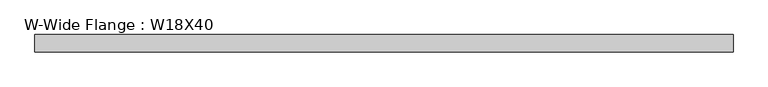
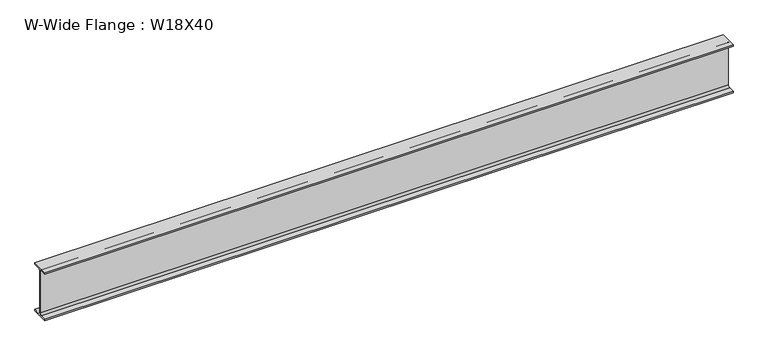
"""IFC4 building model written with IfcOpenShell, lengths in millimetres: beam geometry, W-Wide Flange : W18X40."""

import ifcopenshell
import ifcopenshell.guid

model = None  # the IFC model being written
_history = None  # IfcOwnerHistory: only IFC2X3 demands one
_inside = {}  # id of a spatial element -> (the spatial element, [elements in it])
_under = {}  # id of a project, library or spatial element -> (it, [spatial elements below it])
_declared = {}  # id of a project -> (the project, [libraries it declares])
_typed = {}  # id of a type object -> (the type object, [elements of that type])
_made_of = {}  # id of a material, layer set ... -> (it, [elements and type objects made of it])


def new_model(schema):
    """Start an empty IFC model of exactly this schema.

    Asked for "IFC4X3", IfcOpenShell would pick the latest addendum, in which some entities
    have other attributes; the version numbers below select the first issue.
    IFC2X3 requires an IfcOwnerHistory on every rooted entity: one is made here for all.
    """
    global model, _history
    if schema == "IFC4X3":
        model = ifcopenshell.file(schema_version=(4, 3, 0, 0))
    else:
        model = ifcopenshell.file(schema=schema)
    _inside.clear()
    _under.clear()
    _declared.clear()
    _typed.clear()
    _made_of.clear()
    _history = None
    if model.schema == "IFC2X3":
        org = make("IfcOrganization", Name="unknown")
        user = make(
            "IfcPersonAndOrganization",
            ThePerson=make("IfcPerson", FamilyName="unknown"),
            TheOrganization=org,
        )
        app = make(
            "IfcApplication",
            ApplicationDeveloper=org,
            Version="unknown",
            ApplicationFullName="unknown",
            ApplicationIdentifier="unknown",
        )
        _history = make(
            "IfcOwnerHistory",
            OwningUser=user,
            OwningApplication=app,
            ChangeAction="ADDED",
            CreationDate=0,
        )
    return model


def make(cls, **values):
    """One entity of the class cls with the attributes given. An attribute that is None is left unset."""
    return model.create_entity(
        cls, **{name: value for name, value in values.items() if value is not None}
    )


def rooted(cls, **values):
    """An entity with a GlobalId (a new one), such as an element, a storey or a relation."""
    return make(cls, GlobalId=ifcopenshell.guid.new(), OwnerHistory=_history, **values)


def si_unit(unit_type, name, prefix=None):
    """IfcSIUnit, for example si_unit("LENGTHUNIT", "METRE", prefix="MILLI")."""
    return make("IfcSIUnit", UnitType=unit_type, Prefix=prefix, Name=name)


def assignment(units):
    """IfcUnitAssignment: the units of a project."""
    return None if units is None else make("IfcUnitAssignment", Units=units)


def point(xyz):
    """IfcCartesianPoint."""
    return None if xyz is None else make("IfcCartesianPoint", Coordinates=xyz)


def direction(xyz):
    """IfcDirection."""
    return None if xyz is None else make("IfcDirection", DirectionRatios=xyz)


def frame(location, z_axis=None, x_axis=None):
    """IfcAxis2Placement3D, a coordinate frame: its origin and axes. An axis left out is left unset."""
    return make(
        "IfcAxis2Placement3D",
        Location=point(location),
        Axis=direction(z_axis),
        RefDirection=direction(x_axis),
    )


def frame_2d(location, x_axis=None):
    """IfcAxis2Placement2D, a coordinate frame in the plane: its origin and x axis."""
    return make(
        "IfcAxis2Placement2D", Location=point(location), RefDirection=direction(x_axis)
    )


def origin():
    """The frame at (0, 0, 0) with its axes left unset."""
    return frame((0.0, 0.0, 0.0))


def place(relative_to, where):
    """IfcLocalPlacement: puts the frame where relative to a parent placement (None: the world)."""
    return make(
        "IfcLocalPlacement", PlacementRelTo=relative_to, RelativePlacement=where
    )


def context(
    kind, dimensions, precision=None, world=None, true_north=None, identifier=None
):
    """IfcGeometricRepresentationContext, for example the 3D "Model" context."""
    return make(
        "IfcGeometricRepresentationContext",
        ContextIdentifier=identifier,
        ContextType=kind,
        CoordinateSpaceDimension=dimensions,
        Precision=precision,
        WorldCoordinateSystem=world,
        TrueNorth=true_north,
    )


def project(units=None, contexts=None):
    """IfcProject with its units and contexts."""
    return rooted(
        "IfcProject",
        Name="project",
        RepresentationContexts=contexts,
        UnitsInContext=assignment(units),
    )


def spatial(cls, under=None, at=None, **own):
    """A site, building, storey or space (cls), placed at a placement, below another one or the project."""
    s = rooted(cls, ObjectPlacement=at, **own)
    if under is not None:
        _under.setdefault(under.id(), (under, []))[1].append(s)
    return s


def polyline(points):
    """IfcPolyline through the points."""
    return make("IfcPolyline", Points=[point(p) for p in points])


def circle_curve(where, radius):
    """IfcCircle in the frame where."""
    return make("IfcCircle", Position=where, Radius=radius)


def trimmed(basis, trim1, trim2, sense, master):
    """IfcTrimmedCurve: the piece of a basis curve between two trims."""
    return make(
        "IfcTrimmedCurve",
        BasisCurve=basis,
        Trim1=trim1,
        Trim2=trim2,
        SenseAgreement=sense,
        MasterRepresentation=master,
    )


def segment(curve, same_sense, transition):
    """IfcCompositeCurveSegment."""
    return make(
        "IfcCompositeCurveSegment",
        Transition=transition,
        SameSense=same_sense,
        ParentCurve=curve,
    )


def composite_curve(segments, self_intersect=None):
    """IfcCompositeCurve: segments joined end to end."""
    return make("IfcCompositeCurve", Segments=segments, SelfIntersect=self_intersect)


def outline(outer, holes=None, kind="AREA"):
    """IfcArbitraryClosedProfileDef: a profile drawn as a closed curve; with holes, ...WithVoids."""
    if holes is None:
        return make("IfcArbitraryClosedProfileDef", ProfileType=kind, OuterCurve=outer)
    return make(
        "IfcArbitraryProfileDefWithVoids",
        ProfileType=kind,
        OuterCurve=outer,
        InnerCurves=holes,
    )


def extrude(swept, where, along, depth):
    """IfcExtrudedAreaSolid: the profile swept, set in the frame where, extruded along a direction by depth."""
    return make(
        "IfcExtrudedAreaSolid",
        SweptArea=swept,
        Position=where,
        ExtrudedDirection=direction(along),
        Depth=depth,
    )


def shape(context_of_items, identifier, shape_type, items):
    """IfcShapeRepresentation: the items that make up one representation, for example the "Body"."""
    return make(
        "IfcShapeRepresentation",
        ContextOfItems=context_of_items,
        RepresentationIdentifier=identifier,
        RepresentationType=shape_type,
        Items=items,
    )


def source(mapping_origin, context_of_items, identifier, shape_type, items):
    """IfcRepresentationMap: a shape defined once, which mapped items show again and again."""
    return make(
        "IfcRepresentationMap",
        MappingOrigin=mapping_origin,
        MappedRepresentation=shape(context_of_items, identifier, shape_type, items),
    )


def transform(
    local_origin,
    x_axis=None,
    y_axis=None,
    z_axis=None,
    scale=None,
    scale2=None,
    scale3=None,
    uniform=True,
):
    """IfcCartesianTransformationOperator3D, or its non-uniform kind. x_axis, y_axis, z_axis: its Axis1, 2, 3."""
    if uniform:
        return make(
            "IfcCartesianTransformationOperator3D",
            Axis1=direction(x_axis),
            Axis2=direction(y_axis),
            LocalOrigin=point(local_origin),
            Scale=scale,
            Axis3=direction(z_axis),
        )
    return make(
        "IfcCartesianTransformationOperator3DnonUniform",
        Axis1=direction(x_axis),
        Axis2=direction(y_axis),
        LocalOrigin=point(local_origin),
        Scale=scale,
        Axis3=direction(z_axis),
        Scale2=scale2,
        Scale3=scale3,
    )


def mapped(mapping_source, mapping_target):
    """IfcMappedItem: shows the shape of a source again, moved by a transform."""
    return make(
        "IfcMappedItem", MappingSource=mapping_source, MappingTarget=mapping_target
    )


def made_of(thing, what):
    """Note that an element or type object is made of a material, layer set ...; save() writes the relation."""
    if what is not None:
        _made_of.setdefault(what.id(), (what, []))[1].append(thing)
    return thing


def element(
    cls,
    number,
    at=None,
    inside=None,
    cuts=None,
    type_object=None,
    material=None,
    context=None,
    identifier="Body",
    shape_type=None,
    held_by="IfcProductDefinitionShape",
    body=None,
    shapes=None,
    **own,
):
    """One element of the class cls, such as IfcWall. Its Tag is "e" and its number.

    at: its placement. inside: the storey or other place that contains it. cuts: it is an
    opening in that element (IfcRelVoidsElement). A single representation is given by context,
    identifier, shape_type and body (its items); several are given by shapes. held_by: the class
    of the entity that holds the representations. save() writes the other relations.
    """
    e = rooted(cls, Tag="e%d" % number, ObjectPlacement=at, **own)
    if body is not None:
        shapes = [shape(context, identifier, shape_type, body)]
    if shapes is not None:
        e.Representation = make(held_by, Representations=shapes)
    if inside is not None:
        _inside.setdefault(inside.id(), (inside, []))[1].append(e)
    if cuts is not None:
        rooted(
            "IfcRelVoidsElement", RelatingBuildingElement=cuts, RelatedOpeningElement=e
        )
    if type_object is not None:
        _typed.setdefault(type_object.id(), (type_object, []))[1].append(e)
    return made_of(e, material)


def aggregate(whole, parts):
    """IfcRelAggregates: a whole, such as a stair, and the parts it consists of."""
    return rooted("IfcRelAggregates", RelatingObject=whole, RelatedObjects=parts)


def save(model, path):
    """Write the relations noted so far, then the file.

    IfcRelAggregates (storeys below a building ...), IfcRelContainedInSpatialStructure (elements
    in a storey), IfcRelDefinesByType, IfcRelAssociatesMaterial and IfcRelDeclares: one each for
    every whole, place, type object, material and project.
    """
    for whole, parts in _under.values():
        aggregate(whole, parts)
    for where, things in _inside.values():
        rooted(
            "IfcRelContainedInSpatialStructure",
            RelatedElements=things,
            RelatingStructure=where,
        )
    for kind, things in _typed.values():
        rooted("IfcRelDefinesByType", RelatedObjects=things, RelatingType=kind)
    for what, things in _made_of.values():
        rooted("IfcRelAssociatesMaterial", RelatedObjects=things, RelatingMaterial=what)
    for by, libraries in _declared.values():
        rooted("IfcRelDeclares", RelatingContext=by, RelatedDefinitions=libraries)
    model.write(path)


def w_wide_flange_w18x40_5b02e5c9(model_context):
    return source(origin(), model_context, "Body", "SweptSolid", [
        extrude(outline(composite_curve([segment(polyline([(76.454, -213.995), (76.454, -227.33), (-76.454, -227.33), (-76.454, -213.995), (-20.828, -213.995)]), True, "CONTINUOUS"), segment(trimmed(circle_curve(frame_2d((-20.828, -197.1675)), 16.8275), [point((-20.828, -213.995))], [point((-4.0005, -197.1675))], True, "CARTESIAN"), True, "CONTINUOUS"), segment(polyline([(-4.0005, -197.1675), (-4.0005, 197.1675)]), True, "CONTINUOUS"), segment(trimmed(circle_curve(frame_2d((-20.828, 197.1675)), 16.8275), [point((-4.0005, 197.1675))], [point((-20.828, 213.995))], True, "CARTESIAN"), True, "CONTINUOUS"), segment(polyline([(-20.828, 213.995), (-76.454, 213.995), (-76.454, 227.33), (76.454, 227.33), (76.454, 213.995), (20.828, 213.995)]), True, "CONTINUOUS"), segment(trimmed(circle_curve(frame_2d((20.828, 197.1675)), 16.8275), [point((20.828, 213.995))], [point((4.0005, 197.1675))], True, "CARTESIAN"), True, "CONTINUOUS"), segment(polyline([(4.0005, 197.1675), (4.0005, -197.1675)]), True, "CONTINUOUS"), segment(trimmed(circle_curve(frame_2d((20.828, -197.1675)), 16.8275), [point((4.0005, -197.1675))], [point((20.828, -213.995))], True, "CARTESIAN"), True, "CONTINUOUS"), segment(polyline([(20.828, -213.995), (76.454, -213.995)]), True, "CONTINUOUS")], self_intersect=False)), frame((-3079.75, 0.0, 0.0), z_axis=(1.0, 0.0, 0.0), x_axis=(0.0, 1.0, 0.0)), (0.0, 0.0, 1.0), 6159.5),
    ])


if __name__ == "__main__":
    model = new_model("IFC4")
    model_context = context("Model", 3, world=origin())
    ifc_project = project(units=[si_unit("LENGTHUNIT", "METRE", prefix="MILLI")], contexts=[model_context])
    site = spatial("IfcSite", under=ifc_project)
    building = spatial("IfcBuilding", under=site)
    placement = place(None, origin())
    w_wide_flange_w18x40_shape = w_wide_flange_w18x40_5b02e5c9(model_context)
    element("IfcBeam", 1, ObjectType="W-Wide Flange : W18X40", at=placement, inside=building, context=model_context, shape_type="MappedRepresentation", body=[
        mapped(w_wide_flange_w18x40_shape, transform((0.0, 0.0, 0.0), x_axis=(1.0, 0.0, 0.0), y_axis=(0.0, 1.0, 0.0), z_axis=(0.0, 0.0, 1.0))),
    ])
    save(model, "model.ifc")

# Revit data of these elements
# Type "W-Wide Flange : W18X40"
#   Assembly Code = "B10"
#   W = 40
#   Length [instance default] = 5' - 0"
#   bf = 0' - 6.02"
#   d = 1' - 5.9"
#   k = 0' - 1 3/16"
#   k2 = 0' - 0.6625"
#   tf = 0' - 0.525"
#   tw = 0' - 0.315"
#   A = 0.0819444 SF
#   Structural Material [instance default] = Steel ASTM A992
# Element 1 (IfcBeam, "W-Wide Flange : W18X40")
#   Materials on its faces: "Steel ASTM A992"
# Materials
#   "Steel ASTM A992": class "Metal", colour RGB 199 199 199, transparency 0, Description = "Structural steel 50ksi", Cost = 0
